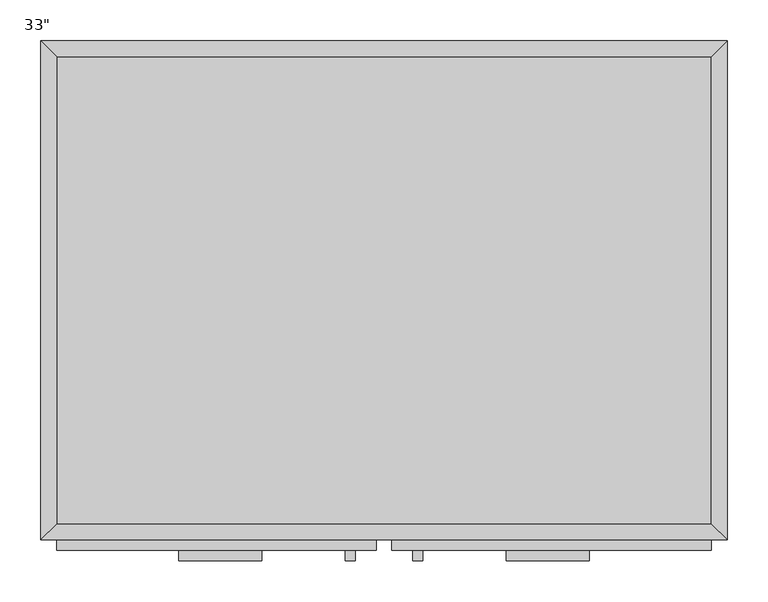
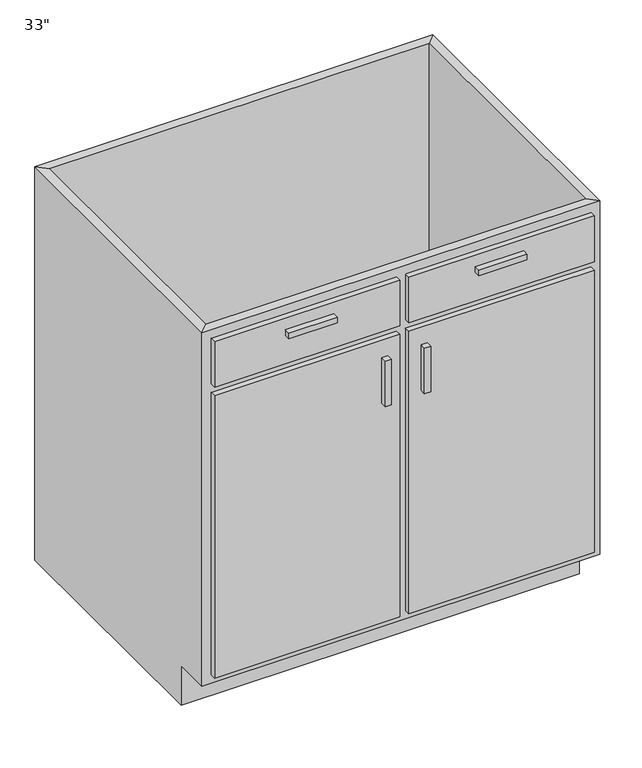
"""IFC4 building model written with IfcOpenShell, lengths in millimetres: furniture geometry."""

import ifcopenshell
import ifcopenshell.guid

model = None  # the IFC model being written
_history = None  # IfcOwnerHistory: only IFC2X3 demands one
_inside = {}  # id of a spatial element -> (the spatial element, [elements in it])
_under = {}  # id of a project, library or spatial element -> (it, [spatial elements below it])
_declared = {}  # id of a project -> (the project, [libraries it declares])
_typed = {}  # id of a type object -> (the type object, [elements of that type])
_made_of = {}  # id of a material, layer set ... -> (it, [elements and type objects made of it])


def new_model(schema):
    """Start an empty IFC model of exactly this schema.

    Asked for "IFC4X3", IfcOpenShell would pick the latest addendum, in which some entities
    have other attributes; the version numbers below select the first issue.
    IFC2X3 requires an IfcOwnerHistory on every rooted entity: one is made here for all.
    """
    global model, _history
    if schema == "IFC4X3":
        model = ifcopenshell.file(schema_version=(4, 3, 0, 0))
    else:
        model = ifcopenshell.file(schema=schema)
    _inside.clear()
    _under.clear()
    _declared.clear()
    _typed.clear()
    _made_of.clear()
    _history = None
    if model.schema == "IFC2X3":
        org = make("IfcOrganization", Name="unknown")
        user = make(
            "IfcPersonAndOrganization",
            ThePerson=make("IfcPerson", FamilyName="unknown"),
            TheOrganization=org,
        )
        app = make(
            "IfcApplication",
            ApplicationDeveloper=org,
            Version="unknown",
            ApplicationFullName="unknown",
            ApplicationIdentifier="unknown",
        )
        _history = make(
            "IfcOwnerHistory",
            OwningUser=user,
            OwningApplication=app,
            ChangeAction="ADDED",
            CreationDate=0,
        )
    return model


def make(cls, **values):
    """One entity of the class cls with the attributes given. An attribute that is None is left unset."""
    return model.create_entity(
        cls, **{name: value for name, value in values.items() if value is not None}
    )


def rooted(cls, **values):
    """An entity with a GlobalId (a new one), such as an element, a storey or a relation."""
    return make(cls, GlobalId=ifcopenshell.guid.new(), OwnerHistory=_history, **values)


def si_unit(unit_type, name, prefix=None):
    """IfcSIUnit, for example si_unit("LENGTHUNIT", "METRE", prefix="MILLI")."""
    return make("IfcSIUnit", UnitType=unit_type, Prefix=prefix, Name=name)


def assignment(units):
    """IfcUnitAssignment: the units of a project."""
    return None if units is None else make("IfcUnitAssignment", Units=units)


def point(xyz):
    """IfcCartesianPoint."""
    return None if xyz is None else make("IfcCartesianPoint", Coordinates=xyz)


def direction(xyz):
    """IfcDirection."""
    return None if xyz is None else make("IfcDirection", DirectionRatios=xyz)


def frame(location, z_axis=None, x_axis=None):
    """IfcAxis2Placement3D, a coordinate frame: its origin and axes. An axis left out is left unset."""
    return make(
        "IfcAxis2Placement3D",
        Location=point(location),
        Axis=direction(z_axis),
        RefDirection=direction(x_axis),
    )


def origin():
    """The frame at (0, 0, 0) with its axes left unset."""
    return frame((0.0, 0.0, 0.0))


def place(relative_to, where):
    """IfcLocalPlacement: puts the frame where relative to a parent placement (None: the world)."""
    return make(
        "IfcLocalPlacement", PlacementRelTo=relative_to, RelativePlacement=where
    )


def context(
    kind, dimensions, precision=None, world=None, true_north=None, identifier=None
):
    """IfcGeometricRepresentationContext, for example the 3D "Model" context."""
    return make(
        "IfcGeometricRepresentationContext",
        ContextIdentifier=identifier,
        ContextType=kind,
        CoordinateSpaceDimension=dimensions,
        Precision=precision,
        WorldCoordinateSystem=world,
        TrueNorth=true_north,
    )


def project(units=None, contexts=None):
    """IfcProject with its units and contexts."""
    return rooted(
        "IfcProject",
        Name="project",
        RepresentationContexts=contexts,
        UnitsInContext=assignment(units),
    )


def spatial(cls, under=None, at=None, **own):
    """A site, building, storey or space (cls), placed at a placement, below another one or the project."""
    s = rooted(cls, ObjectPlacement=at, **own)
    if under is not None:
        _under.setdefault(under.id(), (under, []))[1].append(s)
    return s


def polyline(points):
    """IfcPolyline through the points."""
    return make("IfcPolyline", Points=[point(p) for p in points])


def outline(outer, holes=None, kind="AREA"):
    """IfcArbitraryClosedProfileDef: a profile drawn as a closed curve; with holes, ...WithVoids."""
    if holes is None:
        return make("IfcArbitraryClosedProfileDef", ProfileType=kind, OuterCurve=outer)
    return make(
        "IfcArbitraryProfileDefWithVoids",
        ProfileType=kind,
        OuterCurve=outer,
        InnerCurves=holes,
    )


def extrude(swept, where, along, depth):
    """IfcExtrudedAreaSolid: the profile swept, set in the frame where, extruded along a direction by depth."""
    return make(
        "IfcExtrudedAreaSolid",
        SweptArea=swept,
        Position=where,
        ExtrudedDirection=direction(along),
        Depth=depth,
    )


def faces_of(points, faces, orient=None, outer=None):
    """IfcFace entities. A face is a list of loops; a loop is a list of indices into points, from 0.

    orient and outer hold one flag for each loop. By default every Orientation is true, the
    first loop of a face is its IfcFaceOuterBound and the others are IfcFaceBound.
    """
    made = []
    for i, loops in enumerate(faces):
        bounds = []
        for j, loop in enumerate(loops):
            is_outer = j == 0 if outer is None else outer[i][j]
            bounds.append(
                make(
                    "IfcFaceOuterBound" if is_outer else "IfcFaceBound",
                    Bound=make("IfcPolyLoop", Polygon=[points[k] for k in loop]),
                    Orientation=True if orient is None else orient[i][j],
                )
            )
        made.append(make("IfcFace", Bounds=bounds))
    return made


def faceted_brep(points, faces, orient=None, outer=None, voids=None):
    """IfcFacetedBrep: a solid bounded by flat faces; with voids (closed shells), ...WithVoids."""
    shared = [point(p) for p in points]
    hull = make("IfcClosedShell", CfsFaces=faces_of(shared, faces, orient, outer))
    if voids is None:
        return make("IfcFacetedBrep", Outer=hull)
    return make(
        "IfcFacetedBrepWithVoids",
        Outer=hull,
        Voids=[
            make(cls, CfsFaces=faces_of(shared, fs, o, b)) for cls, fs, o, b in voids
        ],
    )


def shape(context_of_items, identifier, shape_type, items):
    """IfcShapeRepresentation: the items that make up one representation, for example the "Body"."""
    return make(
        "IfcShapeRepresentation",
        ContextOfItems=context_of_items,
        RepresentationIdentifier=identifier,
        RepresentationType=shape_type,
        Items=items,
    )


def source(mapping_origin, context_of_items, identifier, shape_type, items):
    """IfcRepresentationMap: a shape defined once, which mapped items show again and again."""
    return make(
        "IfcRepresentationMap",
        MappingOrigin=mapping_origin,
        MappedRepresentation=shape(context_of_items, identifier, shape_type, items),
    )


def transform(
    local_origin,
    x_axis=None,
    y_axis=None,
    z_axis=None,
    scale=None,
    scale2=None,
    scale3=None,
    uniform=True,
):
    """IfcCartesianTransformationOperator3D, or its non-uniform kind. x_axis, y_axis, z_axis: its Axis1, 2, 3."""
    if uniform:
        return make(
            "IfcCartesianTransformationOperator3D",
            Axis1=direction(x_axis),
            Axis2=direction(y_axis),
            LocalOrigin=point(local_origin),
            Scale=scale,
            Axis3=direction(z_axis),
        )
    return make(
        "IfcCartesianTransformationOperator3DnonUniform",
        Axis1=direction(x_axis),
        Axis2=direction(y_axis),
        LocalOrigin=point(local_origin),
        Scale=scale,
        Axis3=direction(z_axis),
        Scale2=scale2,
        Scale3=scale3,
    )


def mapped(mapping_source, mapping_target):
    """IfcMappedItem: shows the shape of a source again, moved by a transform."""
    return make(
        "IfcMappedItem", MappingSource=mapping_source, MappingTarget=mapping_target
    )


def made_of(thing, what):
    """Note that an element or type object is made of a material, layer set ...; save() writes the relation."""
    if what is not None:
        _made_of.setdefault(what.id(), (what, []))[1].append(thing)
    return thing


def element(
    cls,
    number,
    at=None,
    inside=None,
    cuts=None,
    type_object=None,
    material=None,
    context=None,
    identifier="Body",
    shape_type=None,
    held_by="IfcProductDefinitionShape",
    body=None,
    shapes=None,
    **own,
):
    """One element of the class cls, such as IfcWall. Its Tag is "e" and its number.

    at: its placement. inside: the storey or other place that contains it. cuts: it is an
    opening in that element (IfcRelVoidsElement). A single representation is given by context,
    identifier, shape_type and body (its items); several are given by shapes. held_by: the class
    of the entity that holds the representations. save() writes the other relations.
    """
    e = rooted(cls, Tag="e%d" % number, ObjectPlacement=at, **own)
    if body is not None:
        shapes = [shape(context, identifier, shape_type, body)]
    if shapes is not None:
        e.Representation = make(held_by, Representations=shapes)
    if inside is not None:
        _inside.setdefault(inside.id(), (inside, []))[1].append(e)
    if cuts is not None:
        rooted(
            "IfcRelVoidsElement", RelatingBuildingElement=cuts, RelatedOpeningElement=e
        )
    if type_object is not None:
        _typed.setdefault(type_object.id(), (type_object, []))[1].append(e)
    return made_of(e, material)


def aggregate(whole, parts):
    """IfcRelAggregates: a whole, such as a stair, and the parts it consists of."""
    return rooted("IfcRelAggregates", RelatingObject=whole, RelatedObjects=parts)


def save(model, path):
    """Write the relations noted so far, then the file.

    IfcRelAggregates (storeys below a building ...), IfcRelContainedInSpatialStructure (elements
    in a storey), IfcRelDefinesByType, IfcRelAssociatesMaterial and IfcRelDeclares: one each for
    every whole, place, type object, material and project.
    """
    for whole, parts in _under.values():
        aggregate(whole, parts)
    for where, things in _inside.values():
        rooted(
            "IfcRelContainedInSpatialStructure",
            RelatedElements=things,
            RelatingStructure=where,
        )
    for kind, things in _typed.values():
        rooted("IfcRelDefinesByType", RelatedObjects=things, RelatingType=kind)
    for what, things in _made_of.values():
        rooted("IfcRelAssociatesMaterial", RelatedObjects=things, RelatingMaterial=what)
    for by, libraries in _declared.values():
        rooted("IfcRelDeclares", RelatingContext=by, RelatedDefinitions=libraries)
    model.write(path)


def furniture_7de88fd5(model_context):
    return source(origin(), model_context, "Body", "SolidModel", [
        faceted_brep([(418.7877049, -590.55, 876.3), (418.7877049, -590.55, 88.9), (-381.3122951, -590.55, 88.9), (-381.3122951, -590.55, 876.3), (-400.3622951, -609.6, 876.3), (437.8377049, -609.6, 876.3), (-400.3622951, -609.6, 88.9), (437.8377049, -609.6, 88.9), (-381.3122951, -533.4, 88.9), (-381.3122951, -19.05, 88.9), (-381.3122951, -19.05, 876.3), (-400.3622951, 0.0, 876.3), (-400.3622951, 0.0, 0.0), (-400.3622951, -533.4, 0.0), (-400.3622951, -533.4, 88.9), (418.7877049, -19.05, 88.9), (418.7877049, -19.05, 876.3), (437.8377049, 0.0, 876.3), (437.8377049, 0.0, 0.0), (418.7877049, -533.4, 88.9), (437.8377049, -533.4, 88.9), (437.8377049, -533.4, 0.0)], [[[0, 1, 2, 3]], [[0, 3, 4, 5]], [[5, 4, 6, 7]], [[2, 1, 7, 6]], [[3, 2, 8, 9, 10]], [[4, 3, 10, 11]], [[6, 4, 11, 12, 13, 14]], [[2, 6, 14, 8]], [[10, 9, 15, 16]], [[11, 10, 16, 17]], [[12, 11, 17, 18]], [[1, 0, 16, 15, 19]], [[0, 5, 17, 16]], [[5, 7, 20, 21, 18, 17]], [[7, 1, 19, 20]], [[8, 19, 15, 9]], [[18, 21, 13, 12]], [[13, 21, 20, 19, 8, 14]]]),
        extrude(outline(polyline([(-130.4872951, -635.0), (-232.0872951, -635.0), (-232.0872951, -622.3), (-130.4872951, -622.3), (-130.4872951, -635.0)])), frame((0.0, 0.0, 819.15), z_axis=(0.0, 0.0, 1.0), x_axis=(1.0, 0.0, 0.0)), (0.0, 0.0, 1.0), 12.7),
        extrude(outline(polyline([(269.5627049, -635.0), (167.9627049, -635.0), (167.9627049, -622.3), (269.5627049, -622.3), (269.5627049, -635.0)])), frame((0.0, 0.0, 819.15), z_axis=(0.0, 0.0, 1.0), x_axis=(1.0, 0.0, 0.0)), (0.0, 0.0, 1.0), 12.7),
        extrude(outline(polyline([(-16.1872951, -635.0), (-28.8872951, -635.0), (-28.8872951, -622.3), (-16.1872951, -622.3), (-16.1872951, -635.0)])), frame((0.0, 0.0, 596.9), z_axis=(0.0, 0.0, 1.0), x_axis=(1.0, 0.0, 0.0)), (0.0, 0.0, 1.0), 101.6),
        extrude(outline(polyline([(66.3627049, -635.0), (53.6627049, -635.0), (53.6627049, -622.3), (66.3627049, -622.3), (66.3627049, -635.0)])), frame((0.0, 0.0, 596.9), z_axis=(0.0, 0.0, 1.0), x_axis=(1.0, 0.0, 0.0)), (0.0, 0.0, 1.0), 101.6),
        extrude(outline(polyline([(418.7877049, -19.05), (418.7877049, -590.55), (-381.3122951, -590.55), (-381.3122951, -19.05), (418.7877049, -19.05)])), frame((0.0, 0.0, 88.9), z_axis=(0.0, 0.0, 1.0), x_axis=(1.0, 0.0, 0.0)), (0.0, 0.0, 1.0), 19.05),
        extrude(outline(polyline([(9.2127049, -622.3), (-381.3122951, -622.3), (-381.3122951, -609.6), (9.2127049, -609.6), (9.2127049, -622.3)])), frame((0.0, 0.0, 755.65), z_axis=(0.0, 0.0, 1.0), x_axis=(1.0, 0.0, 0.0)), (0.0, 0.0, 1.0), 101.6),
        extrude(outline(polyline([(418.7877049, -622.3), (28.2627049, -622.3), (28.2627049, -609.6), (418.7877049, -609.6), (418.7877049, -622.3)])), frame((0.0, 0.0, 755.65), z_axis=(0.0, 0.0, 1.0), x_axis=(1.0, 0.0, 0.0)), (0.0, 0.0, 1.0), 101.6),
        extrude(outline(polyline([(9.2127049, -622.3), (-381.3122951, -622.3), (-381.3122951, -609.6), (9.2127049, -609.6), (9.2127049, -622.3)])), frame((0.0, 0.0, 107.95), z_axis=(0.0, 0.0, 1.0), x_axis=(1.0, 0.0, 0.0)), (0.0, 0.0, 1.0), 628.65),
        extrude(outline(polyline([(418.7877049, -622.3), (28.2627049, -622.3), (28.2627049, -609.6), (418.7877049, -609.6), (418.7877049, -622.3)])), frame((0.0, 0.0, 107.95), z_axis=(0.0, 0.0, 1.0), x_axis=(1.0, 0.0, 0.0)), (0.0, 0.0, 1.0), 628.65),
    ])


if __name__ == "__main__":
    model = new_model("IFC4")
    model_context = context("Model", 3, world=origin())
    ifc_project = project(units=[si_unit("LENGTHUNIT", "METRE", prefix="MILLI")], contexts=[model_context])
    site = spatial("IfcSite", under=ifc_project)
    building = spatial("IfcBuilding", under=site)
    placement = place(None, origin())
    furniture_shape = furniture_7de88fd5(model_context)
    element("IfcFurniture", 1, ObjectType="Base Cabinet-Double Door & 2 Drawer : 33\"", at=placement, inside=building, context=model_context, shape_type="MappedRepresentation", body=[
        mapped(furniture_shape, transform((0.0, 0.0, 0.0), x_axis=(1.0, 0.0, 0.0), y_axis=(0.0, 1.0, 0.0), z_axis=(0.0, 0.0, 1.0))),
    ])
    save(model, "model.ifc")

# Revit data of these elements
# Type "Base Cabinet-Double Door & 2 Drawer : 33\""
#   Assembly Code = "C1030410"
#   Depth = 2' - 0"
#   Height = 2' - 10 1/2"
#   Toe Depth = 0' - 3"
#   Toe Height = 0' - 3 1/2"
#   Width = 2' - 9"
#   Cabinet Material = none
#   Door/Drawer Material = none
#   Handle Material = Cabinets - Handles
#   Default Elevation = 0
# Element 1 (IfcFurniture, "Base Cabinet-Double Door & 2 Drawer : 33\"")
#   Materials on its faces: "Cabinets", "Cabinets - Handles"
# Materials
#   "Cabinets - Handles": class "Metal", colour RGB 57 57 57, transparency 0
#   "Cabinets": class "Miscellaneous", colour RGB 249 249 249, transparency 0
